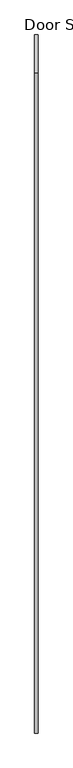
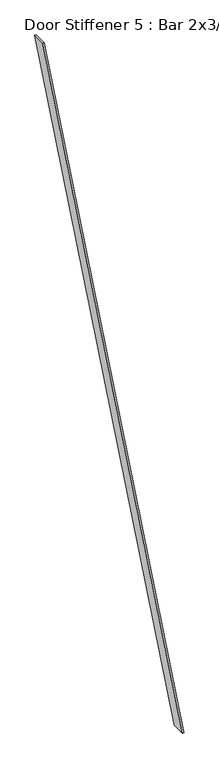
"""IFC4 building model written with IfcOpenShell, lengths in millimetres: proxy geometry, Door Stiffener 5 : Bar 2x3/16."""

from ifc_helpers import new_model, si_unit, frame, origin, place, context, project, spatial, polyline, outline, extrude, source, transform, mapped, element, save


def door_stiffener_5_bar_2x3_16_34f525c1(model_context):
    return source(origin(), model_context, "Body", "SweptSolid", [
        extrude(outline(polyline([(-534200.9077829, 2400.3), (-534145.8788841, 2400.3), (-535108.4374853, 88.9), (-535163.4663841, 88.9), (-534200.9077829, 2400.3)])), frame((587403.9934739, 0.0, 0.0), z_axis=(1.0, 0.0, 0.0), x_axis=(0.0, 1.0, 0.0)), (0.0, 0.0, 1.0), 4.7625),
    ])


if __name__ == "__main__":
    model = new_model("IFC4")
    model_context = context("Model", 3, world=origin())
    ifc_project = project(units=[si_unit("LENGTHUNIT", "METRE", prefix="MILLI")], contexts=[model_context])
    site = spatial("IfcSite", under=ifc_project)
    building = spatial("IfcBuilding", under=site)
    placement = place(None, origin())
    door_stiffener_5_bar_2x3_16_shape = door_stiffener_5_bar_2x3_16_34f525c1(model_context)
    element("IfcBuildingElementProxy", 1, Name="Door Stiffener 5 : Bar 2x3/16", ObjectType="Door Stiffener 5 : Bar 2x3/16", at=placement, inside=building, context=model_context, shape_type="MappedRepresentation", body=[
        mapped(door_stiffener_5_bar_2x3_16_shape, transform((0.0, 0.0, 0.0), x_axis=(1.0, 0.0, 0.0), y_axis=(0.0, 1.0, 0.0), z_axis=(0.0, 0.0, 1.0))),
    ])
    save(model, "model.ifc")

# Revit data of these elements
# Element 1 (IfcBuildingElementProxy, "Door Stiffener 5 : Bar 2x3/16")
#   Materials on its faces: "2\"X3/16\" GALV. STL BAR STOCK"
# Materials
#   "2\"X3/16\" GALV. STL BAR STOCK": class "Generic", colour RGB 211 211 207, transparency 0, Cost = 0
